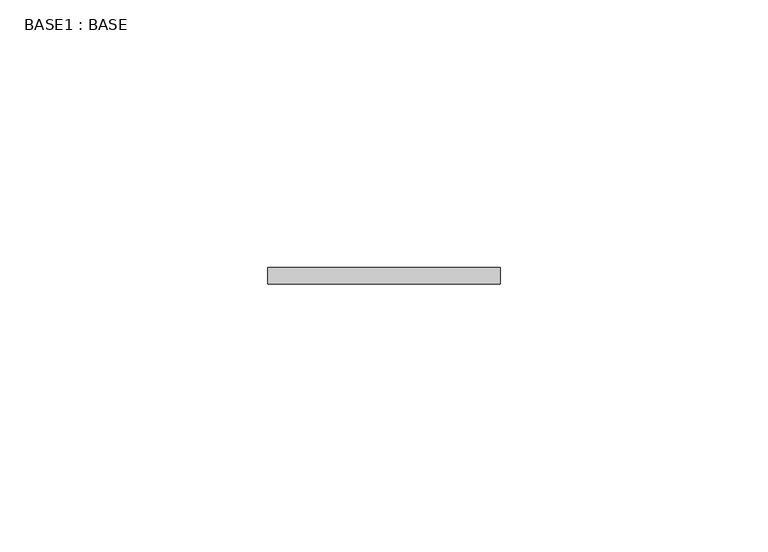
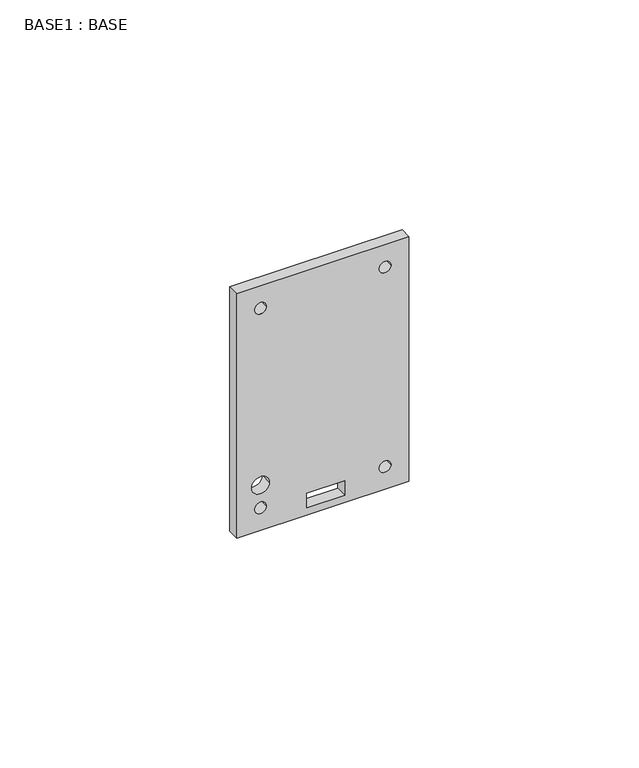
"""IFC4 building model written with IfcOpenShell, lengths in millimetres: proxy geometry, BASE1 : BASE."""

from ifc_helpers import new_model, si_unit, point, frame, frame_2d, origin, place, context, project, spatial, polyline, circle_curve, trimmed, segment, composite_curve, outline, extrude, source, transform, mapped, element, save


def base1_base_8b84c3cf(model_context):
    return source(origin(), model_context, "Body", "SweptSolid", [
        extrude(outline(polyline([(0.0, 2369.0719295), (0.0, 2412.3719295), (65.0, 2412.3719295), (65.0, 2369.0719295), (0.0, 2369.0719295)]), holes=[composite_curve([segment(trimmed(circle_curve(frame_2d((59.0, 2406.3719295)), 1.5), [point((59.0, 2407.8719295))], [point((59.0, 2404.8719295))], True, "CARTESIAN"), True, "CONTINUOUS"), segment(trimmed(circle_curve(frame_2d((59.0, 2406.3719295)), 1.5), [point((59.0, 2404.8719295))], [point((59.0, 2407.8719295))], True, "CARTESIAN"), True, "CONTINUOUS")], self_intersect=False), composite_curve([segment(trimmed(circle_curve(frame_2d((59.0, 2375.0719295)), 1.5), [point((59.0, 2376.5719295))], [point((59.0, 2373.5719295))], True, "CARTESIAN"), True, "CONTINUOUS"), segment(trimmed(circle_curve(frame_2d((59.0, 2375.0719295)), 1.5), [point((59.0, 2373.5719295))], [point((59.0, 2376.5719295))], True, "CARTESIAN"), True, "CONTINUOUS")], self_intersect=False), composite_curve([segment(trimmed(circle_curve(frame_2d((6.0, 2375.0719295)), 1.5), [point((6.0, 2376.5719295))], [point((6.0, 2373.5719295))], True, "CARTESIAN"), True, "CONTINUOUS"), segment(trimmed(circle_curve(frame_2d((6.0, 2375.0719295)), 1.5), [point((6.0, 2373.5719295))], [point((6.0, 2376.5719295))], True, "CARTESIAN"), True, "CONTINUOUS")], self_intersect=False), composite_curve([segment(trimmed(circle_curve(frame_2d((6.0, 2406.3719295)), 1.5), [point((6.0, 2407.8719295))], [point((6.0, 2404.8719295))], True, "CARTESIAN"), True, "CONTINUOUS"), segment(trimmed(circle_curve(frame_2d((6.0, 2406.3719295)), 1.5), [point((6.0, 2404.8719295))], [point((6.0, 2407.8719295))], True, "CARTESIAN"), True, "CONTINUOUS")], self_intersect=False), composite_curve([segment(trimmed(circle_curve(frame_2d((12.0, 2375.0719295)), 2.25), [point((12.0, 2377.3219295))], [point((12.0, 2372.8219295))], True, "CARTESIAN"), True, "CONTINUOUS"), segment(trimmed(circle_curve(frame_2d((12.0, 2375.0719295)), 2.25), [point((12.0, 2372.8219295))], [point((12.0, 2377.3219295))], True, "CARTESIAN"), True, "CONTINUOUS")], self_intersect=False), polyline([(2.0, 2386.6931854), (5.75, 2386.6931854), (5.75, 2396.1931854), (2.0, 2396.1931854), (2.0, 2386.6931854)])]), frame((0.0, 1351.7384159, 0.0), z_axis=(0.0, 1.0, 0.0), x_axis=(0.0, 0.0, 1.0)), (0.0, 0.0, 1.0), 3.0),
    ])


if __name__ == "__main__":
    model = new_model("IFC4")
    model_context = context("Model", 3, world=origin())
    ifc_project = project(units=[si_unit("LENGTHUNIT", "METRE", prefix="MILLI")], contexts=[model_context])
    site = spatial("IfcSite", under=ifc_project)
    building = spatial("IfcBuilding", under=site)
    placement = place(None, origin())
    base1_base_shape = base1_base_8b84c3cf(model_context)
    element("IfcBuildingElementProxy", 1, Name="BASE1 : BASE", ObjectType="BASE1 : BASE", at=placement, inside=building, context=model_context, shape_type="MappedRepresentation", body=[
        mapped(base1_base_shape, transform((0.0, 0.0, 0.0), x_axis=(1.0, 0.0, 0.0), y_axis=(0.0, 1.0, 0.0), z_axis=(0.0, 0.0, 1.0))),
    ])
    save(model, "model.ifc")

# Revit data of these elements
# Element 1 (IfcBuildingElementProxy, "BASE1 : BASE")
#   Materials on its faces: ".BOX FUNDO"
# Materials
#   ".BOX FUNDO": class "Vidro", colour RGB 236 240 239, transparency 0.15, Cost = 0
